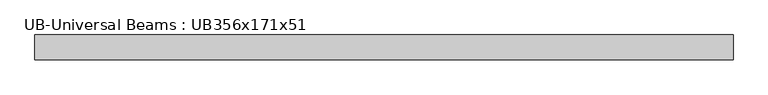
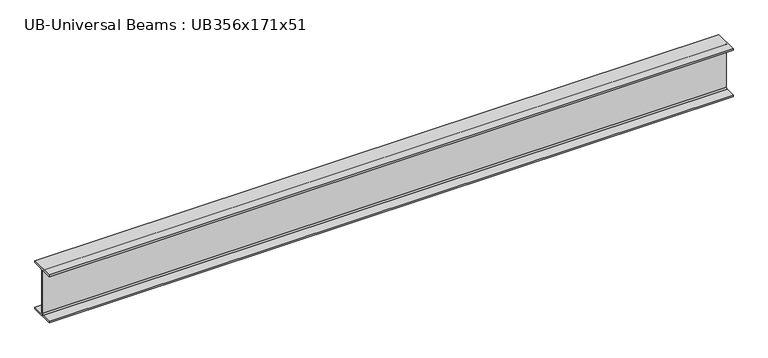
"""IFC4 building model written with IfcOpenShell, lengths in millimetres: beam geometry, UB-Universal Beams : UB356x171x51."""

from ifc_helpers import new_model, si_unit, point, frame, frame_2d, origin, place, context, project, spatial, polyline, circle_curve, trimmed, segment, composite_curve, outline, extrude, source, transform, mapped, element, save


def ub_universal_beams_ub356x171x51_26e98692(model_context):
    return source(origin(), model_context, "Body", "SweptSolid", [
        extrude(outline(composite_curve([segment(polyline([(85.75, -166.0), (85.75, -177.5), (-85.75, -177.5), (-85.75, -166.0), (-13.9, -166.0)]), True, "CONTINUOUS"), segment(trimmed(circle_curve(frame_2d((-13.9, -155.8)), 10.2), [point((-13.9, -166.0))], [point((-3.7, -155.8))], True, "CARTESIAN"), True, "CONTINUOUS"), segment(polyline([(-3.7, -155.8), (-3.7, 155.8)]), True, "CONTINUOUS"), segment(trimmed(circle_curve(frame_2d((-13.9, 155.8)), 10.2), [point((-3.7, 155.8))], [point((-13.9, 166.0))], True, "CARTESIAN"), True, "CONTINUOUS"), segment(polyline([(-13.9, 166.0), (-85.75, 166.0), (-85.75, 177.5), (85.75, 177.5), (85.75, 166.0), (13.9, 166.0)]), True, "CONTINUOUS"), segment(trimmed(circle_curve(frame_2d((13.9, 155.8)), 10.2), [point((13.9, 166.0))], [point((3.7, 155.8))], True, "CARTESIAN"), True, "CONTINUOUS"), segment(polyline([(3.7, 155.8), (3.7, -155.8)]), True, "CONTINUOUS"), segment(trimmed(circle_curve(frame_2d((13.9, -155.8)), 10.2), [point((3.7, -155.8))], [point((13.9, -166.0))], True, "CARTESIAN"), True, "CONTINUOUS"), segment(polyline([(13.9, -166.0), (85.75, -166.0)]), True, "CONTINUOUS")], self_intersect=False)), frame((-2398.3, 0.0, 0.0), z_axis=(1.0, 0.0, 0.0), x_axis=(0.0, 1.0, 0.0)), (0.0, 0.0, 1.0), 4796.6),
    ])


if __name__ == "__main__":
    model = new_model("IFC4")
    model_context = context("Model", 3, world=origin())
    ifc_project = project(units=[si_unit("LENGTHUNIT", "METRE", prefix="MILLI")], contexts=[model_context])
    site = spatial("IfcSite", under=ifc_project)
    building = spatial("IfcBuilding", under=site)
    placement = place(None, origin())
    ub_universal_beams_ub356x171x51_shape = ub_universal_beams_ub356x171x51_26e98692(model_context)
    element("IfcBeam", 1, ObjectType="UB-Universal Beams : UB356x171x51", at=placement, inside=building, context=model_context, shape_type="MappedRepresentation", body=[
        mapped(ub_universal_beams_ub356x171x51_shape, transform((0.0, 0.0, 0.0), x_axis=(1.0, 0.0, 0.0), y_axis=(0.0, 1.0, 0.0), z_axis=(0.0, 0.0, 1.0))),
    ])
    save(model, "model.ifc")

# Revit data of these elements
# Type "UB-Universal Beams : UB356x171x51"
#   Section Name Key = "UB356X171X51"
#   Width = 17.15 cm
#   Web Thickness = 0.74 cm
#   Web Fillet = 1.02 cm
#   Warping Constant = 286000.0 cm⁶
#   Torsional Moment of Inertia = 23.80 cm⁴
#   Section Area = 64.9 cm²
#   Plastic Modulus weak axis = 174.0 cm³
#   Plastic Modulus strong axis = 896.0 cm³
#   Nominal Weight = 50.9998 kgf/m
#   Moment of Inertia weak axis = 968.00 cm⁴
#   Moment of Inertia strong axis = 14136.00 cm⁴
#   Height = 35.5 cm
#   Flange Thickness = 1.15 cm
#   Elastic Modulus weak axis = 113.0 cm³
#   Elastic Modulus strong axis = 796.0 cm³
#   Centroid Vertical = 17.75 cm
#   Centroid Horizontal = 8.575 cm
#   Bolt Spacing = 9.0 cm
#   Length [instance default] = 1500 mm
#   Structural Material [instance default] = Metal - Steel 43-275
#   Type Comments = ""
#   Assembly Code = ""
# Element 1 (IfcBeam, "UB-Universal Beams : UB356x171x51")
#   Materials on its faces: "Metal - Steel 43-275"
# Materials
#   "Metal - Steel 43-275": class "Metal", colour RGB 247 247 247, transparency 0, Cost = 0
